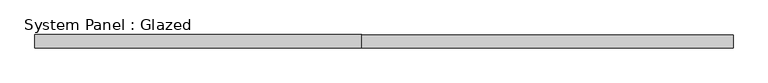
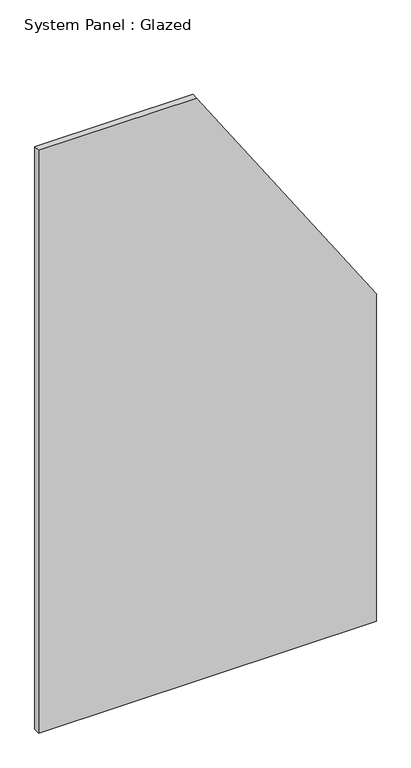
"""IFC4 building model written with IfcOpenShell, lengths in millimetres: plate geometry, System Panel : Glazed."""

from ifc_helpers import new_model, si_unit, frame, origin, place, context, project, spatial, polyline, outline, extrude, source, transform, mapped, element, save


def system_panel_glazed_a7e09480(model_context):
    return source(origin(), model_context, "Body", "SweptSolid", [
        extrude(outline(polyline([(0.0, -658.3333334), (0.0, 658.3333334), (1349.8969043, 658.3333334), (2400.0, -41.8316423), (2400.0, -658.3333334), (0.0, -658.3333334)])), frame((0.0, 24.5, 0.0), z_axis=(0.0, 1.0, 0.0), x_axis=(0.0, 0.0, 1.0)), (0.0, 0.0, 1.0), 25.0),
    ])


if __name__ == "__main__":
    model = new_model("IFC4")
    model_context = context("Model", 3, world=origin())
    ifc_project = project(units=[si_unit("LENGTHUNIT", "METRE", prefix="MILLI")], contexts=[model_context])
    site = spatial("IfcSite", under=ifc_project)
    building = spatial("IfcBuilding", under=site)
    placement = place(None, origin())
    system_panel_glazed_shape = system_panel_glazed_a7e09480(model_context)
    element("IfcPlate", 1, ObjectType="System Panel : Glazed", at=placement, inside=building, context=model_context, shape_type="MappedRepresentation", body=[
        mapped(system_panel_glazed_shape, transform((0.0, 0.0, 0.0), x_axis=(1.0, 0.0, 0.0), y_axis=(0.0, 1.0, 0.0), z_axis=(0.0, 0.0, 1.0))),
    ])
    save(model, "model.ifc")

# Revit data of these elements
# Type "System Panel : Glazed"
#   Keynote = "H11"
#   Construction Type Id = "GSP4R"
#   Analytic Construction = "1/8 in Pilkington single glazing"
#   Visual Light Transmittance = 0.9
#   Solar Heat Gain Coefficient = 0.86
#   Heat Transfer Coefficient (U) = 6.7069 W/(m²·K)
#   Define Thermal Properties by = 1
# Element 1 (IfcPlate, "System Panel : Glazed")
#   Materials on its faces: "Glass"
# Materials
#   "Glass": class "Glass", colour RGB 0 128 192, transparency 0.9, Description = "Soda Lime Glass", Cost = 0
